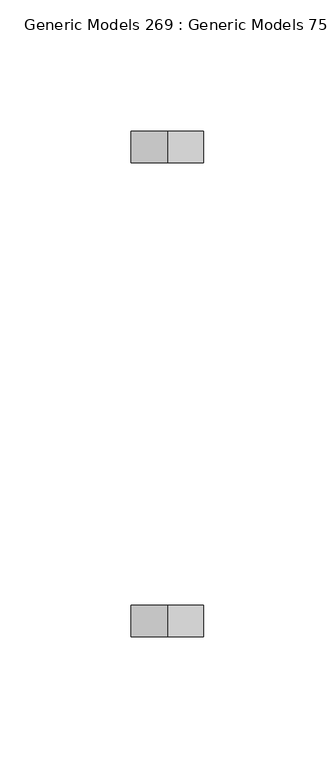
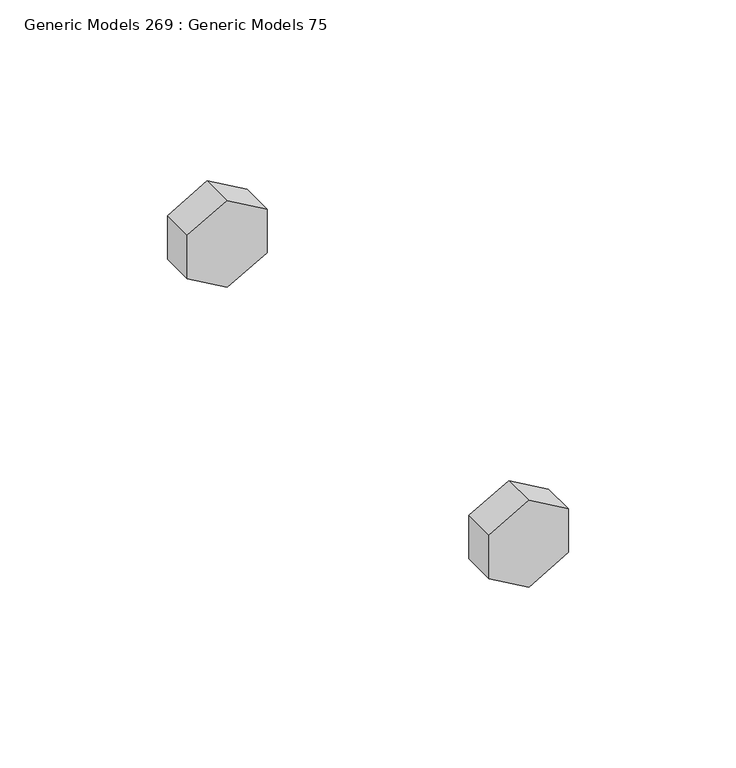
"""IFC4 building model written with IfcOpenShell, lengths in millimetres: proxy geometry, Generic Models 269 : Generic Models 75."""

from ifc_helpers import new_model, si_unit, frame, origin, place, context, project, spatial, polyline, outline, extrude, source, transform, mapped, element, save


def generic_models_269_generic_models_75_3d579b9c(model_context):
    return source(origin(), model_context, "Body", "SweptSolid", [
        extrude(outline(polyline([(268689.2902933, 31975.9942029), (268673.4537198, 31975.9942029), (268665.535433, 31989.7090778), (268673.4537198, 32003.4239528), (268689.2902933, 32003.4239528), (268697.20858, 31989.7090778), (268689.2902933, 31975.9942029)])), frame((0.0, 30858.4781612, 0.0), z_axis=(0.0, 1.0, 0.0), x_axis=(0.0, 0.0, 1.0)), (0.0, 0.0, 1.0), 11.90625),
        extrude(outline(polyline([(268689.2902933, 31975.9942029), (268673.4537198, 31975.9942029), (268665.535433, 31989.7090778), (268673.4537198, 32003.4239528), (268689.2902933, 32003.4239528), (268697.20858, 31989.7090778), (268689.2902933, 31975.9942029)])), frame((0.0, 30678.2969112, 0.0), z_axis=(0.0, 1.0, 0.0), x_axis=(0.0, 0.0, 1.0)), (0.0, 0.0, 1.0), 11.90625),
    ])


if __name__ == "__main__":
    model = new_model("IFC4")
    model_context = context("Model", 3, world=origin())
    ifc_project = project(units=[si_unit("LENGTHUNIT", "METRE", prefix="MILLI")], contexts=[model_context])
    site = spatial("IfcSite", under=ifc_project)
    building = spatial("IfcBuilding", under=site)
    placement = place(None, origin())
    generic_models_269_generic_models_75_shape = generic_models_269_generic_models_75_3d579b9c(model_context)
    element("IfcBuildingElementProxy", 1, Name="Generic Models 269 : Generic Models 75", ObjectType="Generic Models 269 : Generic Models 75", at=placement, inside=building, context=model_context, shape_type="MappedRepresentation", body=[
        mapped(generic_models_269_generic_models_75_shape, transform((0.0, 0.0, 0.0), x_axis=(1.0, 0.0, 0.0), y_axis=(0.0, 1.0, 0.0), z_axis=(0.0, 0.0, 1.0))),
    ])
    save(model, "model.ifc")

# Revit data of these elements
# Element 1 (IfcBuildingElementProxy, "Generic Models 269 : Generic Models 75")
#   Materials on its faces: "3/4\" GALV. THRU BOLTS"
# Materials
#   "3/4\" GALV. THRU BOLTS": class "Generic", colour RGB 105 69 171, transparency 0, Cost = 0
